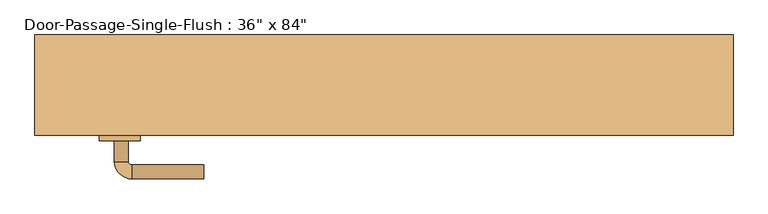
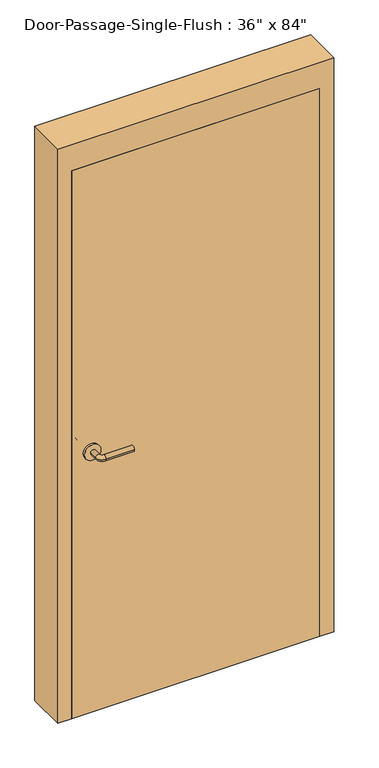
"""IFC4 building model written with IfcOpenShell, lengths in millimetres: door geometry."""

import ifcopenshell
import ifcopenshell.guid

model = None  # the IFC model being written
_history = None  # IfcOwnerHistory: only IFC2X3 demands one
_inside = {}  # id of a spatial element -> (the spatial element, [elements in it])
_under = {}  # id of a project, library or spatial element -> (it, [spatial elements below it])
_declared = {}  # id of a project -> (the project, [libraries it declares])
_typed = {}  # id of a type object -> (the type object, [elements of that type])
_made_of = {}  # id of a material, layer set ... -> (it, [elements and type objects made of it])


def new_model(schema):
    """Start an empty IFC model of exactly this schema.

    Asked for "IFC4X3", IfcOpenShell would pick the latest addendum, in which some entities
    have other attributes; the version numbers below select the first issue.
    IFC2X3 requires an IfcOwnerHistory on every rooted entity: one is made here for all.
    """
    global model, _history
    if schema == "IFC4X3":
        model = ifcopenshell.file(schema_version=(4, 3, 0, 0))
    else:
        model = ifcopenshell.file(schema=schema)
    _inside.clear()
    _under.clear()
    _declared.clear()
    _typed.clear()
    _made_of.clear()
    _history = None
    if model.schema == "IFC2X3":
        org = make("IfcOrganization", Name="unknown")
        user = make(
            "IfcPersonAndOrganization",
            ThePerson=make("IfcPerson", FamilyName="unknown"),
            TheOrganization=org,
        )
        app = make(
            "IfcApplication",
            ApplicationDeveloper=org,
            Version="unknown",
            ApplicationFullName="unknown",
            ApplicationIdentifier="unknown",
        )
        _history = make(
            "IfcOwnerHistory",
            OwningUser=user,
            OwningApplication=app,
            ChangeAction="ADDED",
            CreationDate=0,
        )
    return model


def make(cls, **values):
    """One entity of the class cls with the attributes given. An attribute that is None is left unset."""
    return model.create_entity(
        cls, **{name: value for name, value in values.items() if value is not None}
    )


def rooted(cls, **values):
    """An entity with a GlobalId (a new one), such as an element, a storey or a relation."""
    return make(cls, GlobalId=ifcopenshell.guid.new(), OwnerHistory=_history, **values)


def si_unit(unit_type, name, prefix=None):
    """IfcSIUnit, for example si_unit("LENGTHUNIT", "METRE", prefix="MILLI")."""
    return make("IfcSIUnit", UnitType=unit_type, Prefix=prefix, Name=name)


def assignment(units):
    """IfcUnitAssignment: the units of a project."""
    return None if units is None else make("IfcUnitAssignment", Units=units)


def point(xyz):
    """IfcCartesianPoint."""
    return None if xyz is None else make("IfcCartesianPoint", Coordinates=xyz)


def direction(xyz):
    """IfcDirection."""
    return None if xyz is None else make("IfcDirection", DirectionRatios=xyz)


def frame(location, z_axis=None, x_axis=None):
    """IfcAxis2Placement3D, a coordinate frame: its origin and axes. An axis left out is left unset."""
    return make(
        "IfcAxis2Placement3D",
        Location=point(location),
        Axis=direction(z_axis),
        RefDirection=direction(x_axis),
    )


def frame_2d(location, x_axis=None):
    """IfcAxis2Placement2D, a coordinate frame in the plane: its origin and x axis."""
    return make(
        "IfcAxis2Placement2D", Location=point(location), RefDirection=direction(x_axis)
    )


def origin():
    """The frame at (0, 0, 0) with its axes left unset."""
    return frame((0.0, 0.0, 0.0))


def origin_with_axes():
    """The frame at (0, 0, 0) with the z axis (0, 0, 1) and the x axis (1, 0, 0) written out."""
    return frame((0.0, 0.0, 0.0), z_axis=(0.0, 0.0, 1.0), x_axis=(1.0, 0.0, 0.0))


def place(relative_to, where):
    """IfcLocalPlacement: puts the frame where relative to a parent placement (None: the world)."""
    return make(
        "IfcLocalPlacement", PlacementRelTo=relative_to, RelativePlacement=where
    )


def context(
    kind, dimensions, precision=None, world=None, true_north=None, identifier=None
):
    """IfcGeometricRepresentationContext, for example the 3D "Model" context."""
    return make(
        "IfcGeometricRepresentationContext",
        ContextIdentifier=identifier,
        ContextType=kind,
        CoordinateSpaceDimension=dimensions,
        Precision=precision,
        WorldCoordinateSystem=world,
        TrueNorth=true_north,
    )


def project(units=None, contexts=None):
    """IfcProject with its units and contexts."""
    return rooted(
        "IfcProject",
        Name="project",
        RepresentationContexts=contexts,
        UnitsInContext=assignment(units),
    )


def spatial(cls, under=None, at=None, **own):
    """A site, building, storey or space (cls), placed at a placement, below another one or the project."""
    s = rooted(cls, ObjectPlacement=at, **own)
    if under is not None:
        _under.setdefault(under.id(), (under, []))[1].append(s)
    return s


def polyline(points):
    """IfcPolyline through the points."""
    return make("IfcPolyline", Points=[point(p) for p in points])


def circle_curve(where, radius):
    """IfcCircle in the frame where."""
    return make("IfcCircle", Position=where, Radius=radius)


def ellipse_curve(where, semi_axis1, semi_axis2):
    """IfcEllipse in the frame where."""
    return make(
        "IfcEllipse", Position=where, SemiAxis1=semi_axis1, SemiAxis2=semi_axis2
    )


def trimmed(basis, trim1, trim2, sense, master):
    """IfcTrimmedCurve: the piece of a basis curve between two trims."""
    return make(
        "IfcTrimmedCurve",
        BasisCurve=basis,
        Trim1=trim1,
        Trim2=trim2,
        SenseAgreement=sense,
        MasterRepresentation=master,
    )


def segment(curve, same_sense, transition):
    """IfcCompositeCurveSegment."""
    return make(
        "IfcCompositeCurveSegment",
        Transition=transition,
        SameSense=same_sense,
        ParentCurve=curve,
    )


def composite_curve(segments, self_intersect=None):
    """IfcCompositeCurve: segments joined end to end."""
    return make("IfcCompositeCurve", Segments=segments, SelfIntersect=self_intersect)


def outline(outer, holes=None, kind="AREA"):
    """IfcArbitraryClosedProfileDef: a profile drawn as a closed curve; with holes, ...WithVoids."""
    if holes is None:
        return make("IfcArbitraryClosedProfileDef", ProfileType=kind, OuterCurve=outer)
    return make(
        "IfcArbitraryProfileDefWithVoids",
        ProfileType=kind,
        OuterCurve=outer,
        InnerCurves=holes,
    )


def extrude(swept, where, along, depth):
    """IfcExtrudedAreaSolid: the profile swept, set in the frame where, extruded along a direction by depth."""
    return make(
        "IfcExtrudedAreaSolid",
        SweptArea=swept,
        Position=where,
        ExtrudedDirection=direction(along),
        Depth=depth,
    )


def faces_of(points, faces, orient=None, outer=None):
    """IfcFace entities. A face is a list of loops; a loop is a list of indices into points, from 0.

    orient and outer hold one flag for each loop. By default every Orientation is true, the
    first loop of a face is its IfcFaceOuterBound and the others are IfcFaceBound.
    """
    made = []
    for i, loops in enumerate(faces):
        bounds = []
        for j, loop in enumerate(loops):
            is_outer = j == 0 if outer is None else outer[i][j]
            bounds.append(
                make(
                    "IfcFaceOuterBound" if is_outer else "IfcFaceBound",
                    Bound=make("IfcPolyLoop", Polygon=[points[k] for k in loop]),
                    Orientation=True if orient is None else orient[i][j],
                )
            )
        made.append(make("IfcFace", Bounds=bounds))
    return made


def faceted_brep(points, faces, orient=None, outer=None, voids=None):
    """IfcFacetedBrep: a solid bounded by flat faces; with voids (closed shells), ...WithVoids."""
    shared = [point(p) for p in points]
    hull = make("IfcClosedShell", CfsFaces=faces_of(shared, faces, orient, outer))
    if voids is None:
        return make("IfcFacetedBrep", Outer=hull)
    return make(
        "IfcFacetedBrepWithVoids",
        Outer=hull,
        Voids=[
            make(cls, CfsFaces=faces_of(shared, fs, o, b)) for cls, fs, o, b in voids
        ],
    )


def shape(context_of_items, identifier, shape_type, items):
    """IfcShapeRepresentation: the items that make up one representation, for example the "Body"."""
    return make(
        "IfcShapeRepresentation",
        ContextOfItems=context_of_items,
        RepresentationIdentifier=identifier,
        RepresentationType=shape_type,
        Items=items,
    )


def source(mapping_origin, context_of_items, identifier, shape_type, items):
    """IfcRepresentationMap: a shape defined once, which mapped items show again and again."""
    return make(
        "IfcRepresentationMap",
        MappingOrigin=mapping_origin,
        MappedRepresentation=shape(context_of_items, identifier, shape_type, items),
    )


def transform(
    local_origin,
    x_axis=None,
    y_axis=None,
    z_axis=None,
    scale=None,
    scale2=None,
    scale3=None,
    uniform=True,
):
    """IfcCartesianTransformationOperator3D, or its non-uniform kind. x_axis, y_axis, z_axis: its Axis1, 2, 3."""
    if uniform:
        return make(
            "IfcCartesianTransformationOperator3D",
            Axis1=direction(x_axis),
            Axis2=direction(y_axis),
            LocalOrigin=point(local_origin),
            Scale=scale,
            Axis3=direction(z_axis),
        )
    return make(
        "IfcCartesianTransformationOperator3DnonUniform",
        Axis1=direction(x_axis),
        Axis2=direction(y_axis),
        LocalOrigin=point(local_origin),
        Scale=scale,
        Axis3=direction(z_axis),
        Scale2=scale2,
        Scale3=scale3,
    )


def mapped(mapping_source, mapping_target):
    """IfcMappedItem: shows the shape of a source again, moved by a transform."""
    return make(
        "IfcMappedItem", MappingSource=mapping_source, MappingTarget=mapping_target
    )


def made_of(thing, what):
    """Note that an element or type object is made of a material, layer set ...; save() writes the relation."""
    if what is not None:
        _made_of.setdefault(what.id(), (what, []))[1].append(thing)
    return thing


def element(
    cls,
    number,
    at=None,
    inside=None,
    cuts=None,
    type_object=None,
    material=None,
    context=None,
    identifier="Body",
    shape_type=None,
    held_by="IfcProductDefinitionShape",
    body=None,
    shapes=None,
    **own,
):
    """One element of the class cls, such as IfcWall. Its Tag is "e" and its number.

    at: its placement. inside: the storey or other place that contains it. cuts: it is an
    opening in that element (IfcRelVoidsElement). A single representation is given by context,
    identifier, shape_type and body (its items); several are given by shapes. held_by: the class
    of the entity that holds the representations. save() writes the other relations.
    """
    e = rooted(cls, Tag="e%d" % number, ObjectPlacement=at, **own)
    if body is not None:
        shapes = [shape(context, identifier, shape_type, body)]
    if shapes is not None:
        e.Representation = make(held_by, Representations=shapes)
    if inside is not None:
        _inside.setdefault(inside.id(), (inside, []))[1].append(e)
    if cuts is not None:
        rooted(
            "IfcRelVoidsElement", RelatingBuildingElement=cuts, RelatedOpeningElement=e
        )
    if type_object is not None:
        _typed.setdefault(type_object.id(), (type_object, []))[1].append(e)
    return made_of(e, material)


def aggregate(whole, parts):
    """IfcRelAggregates: a whole, such as a stair, and the parts it consists of."""
    return rooted("IfcRelAggregates", RelatingObject=whole, RelatedObjects=parts)


def save(model, path):
    """Write the relations noted so far, then the file.

    IfcRelAggregates (storeys below a building ...), IfcRelContainedInSpatialStructure (elements
    in a storey), IfcRelDefinesByType, IfcRelAssociatesMaterial and IfcRelDeclares: one each for
    every whole, place, type object, material and project.
    """
    for whole, parts in _under.values():
        aggregate(whole, parts)
    for where, things in _inside.values():
        rooted(
            "IfcRelContainedInSpatialStructure",
            RelatedElements=things,
            RelatingStructure=where,
        )
    for kind, things in _typed.values():
        rooted("IfcRelDefinesByType", RelatedObjects=things, RelatingType=kind)
    for what, things in _made_of.values():
        rooted("IfcRelAssociatesMaterial", RelatedObjects=things, RelatingMaterial=what)
    for by, libraries in _declared.values():
        rooted("IfcRelDeclares", RelatingContext=by, RelatedDefinitions=libraries)
    model.write(path)


def plane_surface(at):
    """IfcPlane: the flat surface through the origin of the frame at, square to its z axis."""
    return make("IfcPlane", Position=at)


def cylinder_surface(at, radius):
    """IfcCylindricalSurface: all points at the distance radius from the z axis of the frame at."""
    return make("IfcCylindricalSurface", Position=at, Radius=radius)


def revolved_surface(curve, axis_point, axis_direction):
    """IfcSurfaceOfRevolution: the curve turned about the line through axis_point along axis_direction."""
    return make(
        "IfcSurfaceOfRevolution",
        SweptCurve=make("IfcArbitraryOpenProfileDef", ProfileType="CURVE", Curve=curve),
        AxisPosition=make("IfcAxis1Placement", Location=point(axis_point), Axis=direction(axis_direction)),
    )


def advanced_brep(points, edges, surfaces, faces):
    """IfcAdvancedBrep: a solid bounded by faces that lie on surfaces and meet in shared edges.

    An edge is (start, end): straight between two places in points (the first is 0);
    or (start, end, curve); or (start, end, curve, False) where it runs against its curve.
    A face is (place in surfaces, loops), or (place, loops, False) where it looks against
    its surface's normal. A loop lists edges by number (the first is 1), with a minus sign
    where the edge is run from its end to its start. The first loop is the outer one.
    """
    corners = [point(p) for p in points]
    vertices = [make("IfcVertexPoint", VertexGeometry=c) for c in corners]
    made = []
    for start, end, *more in edges:
        made.append(
            make(
                "IfcEdgeCurve",
                EdgeStart=vertices[start],
                EdgeEnd=vertices[end],
                EdgeGeometry=more[0] if more else make("IfcPolyline", Points=[corners[start], corners[end]]),
                SameSense=more[1] if len(more) > 1 else True,
            )
        )
    hull = []
    for where, loops, *sense in faces:
        bounds = []
        for j, loop in enumerate(loops):
            ring = [make("IfcOrientedEdge", EdgeElement=made[abs(k) - 1], Orientation=k > 0) for k in loop]
            bounds.append(
                make(
                    "IfcFaceOuterBound" if j == 0 else "IfcFaceBound",
                    Bound=make("IfcEdgeLoop", EdgeList=ring),
                    Orientation=True,
                )
            )
        hull.append(make("IfcAdvancedFace", Bounds=bounds, FaceSurface=surfaces[where], SameSense=sense[0] if sense else True))
    return make("IfcAdvancedBrep", Outer=make("IfcClosedShell", CfsFaces=hull))


def door_01a91e93(model_context):
    return source(origin(), model_context, "Body", "SolidModel", [
        advanced_brep(
        [(-392.190625, -96.775, 1016.0), (-372.190625, -96.775, 1016.0), (-392.190625, -66.775, 1016.0), (-372.190625, -66.775, 1016.0), (-367.190625, -61.775, 1016.0), (-367.190625, -41.775, 1016.0), (-262.190625, -41.775, 1016.0), (-262.190625, -61.775, 1016.0)],
        [
            (0, 1, circle_curve(frame((-382.190625, -96.775, 1016.0), z_axis=(0.0, -1.0, 0.0), x_axis=(1.0, 0.0, 0.0)), 10.0)),
            (1, 0, circle_curve(frame((-382.190625, -96.775, 1016.0), z_axis=(0.0, -1.0, 0.0), x_axis=(1.0, 0.0, 0.0)), 10.0)),
            (0, 2),
            (2, 3, circle_curve(frame((-382.190625, -66.775, 1016.0), z_axis=(0.0, -1.0, 0.0), x_axis=(1.0, 0.0, 0.0)), 10.0)),
            (3, 1),
            (3, 2, circle_curve(frame((-382.190625, -66.775, 1016.0), z_axis=(0.0, -1.0, 0.0), x_axis=(1.0, 0.0, 0.0)), 10.0)),
            (4, 3, circle_curve(frame((-367.190625, -66.775, 1016.0), z_axis=(0.0, 0.0, 1.0), x_axis=(-1.0, 0.0, 0.0)), 5.0)),
            (2, 5, circle_curve(frame((-367.190625, -66.775, 1016.0), z_axis=(0.0, 0.0, -1.0), x_axis=(-1.0, 0.0, 0.0)), 25.0)),
            (5, 4, circle_curve(frame((-367.190625, -51.775, 1016.0), z_axis=(-1.0, 0.0, 0.0), x_axis=(0.0, -1.0, 0.0)), 10.0)),
            (4, 5, circle_curve(frame((-367.190625, -51.775, 1016.0), z_axis=(-1.0, 0.0, 0.0), x_axis=(0.0, -1.0, 0.0)), 10.0)),
            (6, 7, circle_curve(frame((-262.190625, -51.775, 1016.0), z_axis=(1.0, 0.0, 0.0), x_axis=(0.0, -1.0, 0.0)), 10.0)),
            (7, 6, circle_curve(frame((-262.190625, -51.775, 1016.0), z_axis=(1.0, 0.0, 0.0), x_axis=(0.0, -1.0, 0.0)), 10.0)),
            (5, 6),
            (7, 4),
        ],
        [
            plane_surface(frame((-382.190625, -96.775, 1016.0), z_axis=(0.0, -1.0, 0.0), x_axis=(0.0, 0.0, 1.0))),
            cylinder_surface(frame((-382.190625, -96.775, 1016.0), z_axis=(0.0, -1.0, 0.0), x_axis=(1.0, 0.0, 0.0)), 10.0),
            revolved_surface(trimmed(ellipse_curve(frame((-382.190625, -66.775, 1016.0), z_axis=(0.0, -1.0, 0.0), x_axis=(1.0, 0.0, 0.0)), 10.0, 10.0), [point((-392.190625, -66.775, 1016.0))], [point((-372.190625, -66.775, 1016.0))], True, "CARTESIAN"), (-367.190625, -66.775, 1016.0), (0.0, 0.0, -1.0)),
            revolved_surface(trimmed(ellipse_curve(frame((-382.190625, -66.775, 1016.0), z_axis=(0.0, -1.0, 0.0), x_axis=(1.0, 0.0, 0.0)), 10.0, 10.0), [point((-372.190625, -66.775, 1016.0))], [point((-392.190625, -66.775, 1016.0))], True, "CARTESIAN"), (-367.190625, -66.775, 1016.0), (0.0, 0.0, -1.0)),
            plane_surface(frame((-262.190625, -51.775, 1016.0), z_axis=(1.0, 0.0, 0.0), x_axis=(0.0, 0.0, 1.0))),
            cylinder_surface(frame((-367.190625, -51.775, 1016.0), z_axis=(-1.0, 0.0, 0.0), x_axis=(0.0, -1.0, 0.0)), 10.0),
        ],
        [
            (0, [[1, 2]]),
            (1, [[-1, 3, 4, 5]]),
            (1, [[-2, -5, 6, -3]]),
            (2, [[7, -4, 8, 9]]),
            (3, [[-8, -6, -7, 10]]),
            (4, [[11, 12]]),
            (5, [[-9, 13, -12, 14]]),
            (5, [[-10, -14, -11, -13]]),
        ],
    ),
        extrude(outline(composite_curve([segment(trimmed(circle_curve(frame_2d((1016.0, -384.690625)), 30.0), [point((1016.0, -414.690625))], [point((1016.0, -354.690625))], False, "CARTESIAN"), True, "CONTINUOUS"), segment(trimmed(circle_curve(frame_2d((1016.0, -384.690625)), 30.0), [point((1016.0, -354.690625))], [point((1016.0, -414.690625))], False, "CARTESIAN"), True, "CONTINUOUS")], self_intersect=False)), frame((0.0, -104.775, 0.0), z_axis=(0.0, 1.0, 0.0), x_axis=(0.0, 0.0, 1.0)), (0.0, 0.0, 1.0), 8.0),
        advanced_brep(
        [(-392.190625, -157.225, 1016.0), (-372.190625, -157.225, 1016.0), (-372.190625, -187.225, 1016.0), (-392.190625, -187.225, 1016.0), (-367.190625, -192.225, 1016.0), (-367.190625, -212.225, 1016.0), (-262.190625, -212.225, 1016.0), (-262.190625, -192.225, 1016.0)],
        [
            (0, 1, circle_curve(frame((-382.190625, -157.225, 1016.0), z_axis=(0.0, 1.0, 0.0), x_axis=(1.0, 0.0, 0.0)), 10.0)),
            (1, 0, circle_curve(frame((-382.190625, -157.225, 1016.0), z_axis=(0.0, 1.0, 0.0), x_axis=(1.0, 0.0, 0.0)), 10.0)),
            (1, 2),
            (2, 3, circle_curve(frame((-382.190625, -187.225, 1016.0), z_axis=(0.0, 1.0, 0.0), x_axis=(1.0, 0.0, 0.0)), 10.0)),
            (3, 0),
            (3, 2, circle_curve(frame((-382.190625, -187.225, 1016.0), z_axis=(0.0, 1.0, 0.0), x_axis=(1.0, 0.0, 0.0)), 10.0)),
            (4, 5, circle_curve(frame((-367.190625, -202.225, 1016.0), z_axis=(-1.0, 0.0, 0.0), x_axis=(0.0, 1.0, 0.0)), 10.0)),
            (5, 3, circle_curve(frame((-367.190625, -187.225, 1016.0), z_axis=(0.0, 0.0, -1.0), x_axis=(-1.0, 0.0, 0.0)), 25.0)),
            (2, 4, circle_curve(frame((-367.190625, -187.225, 1016.0), z_axis=(0.0, 0.0, 1.0), x_axis=(-1.0, 0.0, 0.0)), 5.0)),
            (5, 4, circle_curve(frame((-367.190625, -202.225, 1016.0), z_axis=(-1.0, 0.0, 0.0), x_axis=(0.0, 1.0, 0.0)), 10.0)),
            (6, 7, circle_curve(frame((-262.190625, -202.225, 1016.0), z_axis=(1.0, 0.0, 0.0), x_axis=(0.0, 1.0, 0.0)), 10.0)),
            (7, 6, circle_curve(frame((-262.190625, -202.225, 1016.0), z_axis=(1.0, 0.0, 0.0), x_axis=(0.0, 1.0, 0.0)), 10.0)),
            (4, 7),
            (6, 5),
        ],
        [
            plane_surface(frame((-382.190625, -157.225, 1016.0), z_axis=(0.0, 1.0, 0.0), x_axis=(0.0, 0.0, 1.0))),
            cylinder_surface(frame((-382.190625, -157.225, 1016.0), z_axis=(0.0, 1.0, 0.0), x_axis=(1.0, 0.0, 0.0)), 10.0),
            revolved_surface(trimmed(ellipse_curve(frame((-382.190625, -187.225, 1016.0), z_axis=(0.0, -1.0, 0.0), x_axis=(1.0, 0.0, 0.0)), 10.0, 10.0), [point((-392.190625, -187.225, 1016.0))], [point((-372.190625, -187.225, 1016.0))], True, "CARTESIAN"), (-367.190625, -187.225, 1016.0), (0.0, 0.0, -1.0)),
            revolved_surface(trimmed(ellipse_curve(frame((-382.190625, -187.225, 1016.0), z_axis=(0.0, -1.0, 0.0), x_axis=(1.0, 0.0, 0.0)), 10.0, 10.0), [point((-372.190625, -187.225, 1016.0))], [point((-392.190625, -187.225, 1016.0))], True, "CARTESIAN"), (-367.190625, -187.225, 1016.0), (0.0, 0.0, -1.0)),
            plane_surface(frame((-262.190625, -202.225, 1016.0), z_axis=(1.0, 0.0, 0.0), x_axis=(0.0, 0.0, 1.0))),
            cylinder_surface(frame((-367.190625, -202.225, 1016.0), z_axis=(-1.0, 0.0, 0.0), x_axis=(0.0, 1.0, 0.0)), 10.0),
        ],
        [
            (0, [[1, 2]]),
            (1, [[3, 4, 5, -2]]),
            (1, [[-5, 6, -3, -1]]),
            (2, [[7, 8, -4, 9]]),
            (3, [[10, -9, -6, -8]]),
            (4, [[11, 12]]),
            (5, [[13, -11, 14, -7]]),
            (5, [[-14, -12, -13, -10]]),
        ],
    ),
        extrude(outline(composite_curve([segment(trimmed(circle_curve(frame_2d((1016.0, -384.690625)), 30.0), [point((1016.0, -414.690625))], [point((1016.0, -354.690625))], False, "CARTESIAN"), True, "CONTINUOUS"), segment(trimmed(circle_curve(frame_2d((1016.0, -384.690625)), 30.0), [point((1016.0, -354.690625))], [point((1016.0, -414.690625))], False, "CARTESIAN"), True, "CONTINUOUS")], self_intersect=False)), frame((0.0, -157.225, 0.0), z_axis=(0.0, 1.0, 0.0), x_axis=(0.0, 0.0, 1.0)), (0.0, 0.0, 1.0), 8.0),
        faceted_brep([(457.2, -100.0125, 0.0), (441.325, -100.0125, 0.0), (441.325, -52.3875, 0.0), (457.2, -52.3875, 0.0), (457.2, -3.175, 0.0), (508.0, -3.175, 0.0), (508.0, -149.225, 0.0), (457.2, -149.225, 0.0), (457.2, -149.225, 2133.6), (457.2, -100.0125, 2133.6), (508.0, -149.225, 2235.2), (-508.0, -149.225, 2235.2), (-508.0, -149.225, 0.0), (-457.2, -149.225, 0.0), (-457.2, -149.225, 2133.6), (508.0, -3.175, 2235.2), (457.2, -3.175, 2133.6), (-457.2, -3.175, 2133.6), (-457.2, -3.175, 0.0), (-508.0, -3.175, 0.0), (-508.0, -3.175, 2235.2), (457.2, -52.3875, 2133.6), (441.325, -52.3875, 2117.725), (-441.325, -52.3875, 2117.725), (-441.325, -52.3875, 0.0), (-457.2, -52.3875, 0.0), (-457.2, -52.3875, 2133.6), (441.325, -100.0125, 2117.725), (-457.2, -100.0125, 2133.6), (-457.2, -100.0125, 0.0), (-441.325, -100.0125, 0.0), (-441.325, -100.0125, 2117.725)], [[[0, 1, 2, 3, 4, 5, 6, 7]], [[7, 8, 9, 0]], [[6, 10, 11, 12, 13, 14, 8, 7]], [[5, 15, 10, 6]], [[4, 16, 17, 18, 19, 20, 15, 5]], [[3, 21, 16, 4]], [[2, 22, 23, 24, 25, 26, 21, 3]], [[1, 27, 22, 2]], [[0, 9, 28, 29, 30, 31, 27, 1]], [[8, 14, 28, 9]], [[16, 21, 26, 17]], [[22, 27, 31, 23]], [[12, 19, 18, 25, 24, 30, 29, 13]], [[13, 29, 28, 14]], [[11, 20, 19, 12]], [[17, 26, 25, 18]], [[23, 31, 30, 24]], [[15, 20, 11, 10]]]),
        extrude(outline(polyline([(457.2, -104.775), (457.2, -149.225), (-457.2, -149.225), (-457.2, -104.775), (457.2, -104.775)])), origin_with_axes(), (0.0, 0.0, 1.0), 2133.6),
    ])


if __name__ == "__main__":
    model = new_model("IFC4")
    model_context = context("Model", 3, world=origin())
    ifc_project = project(units=[si_unit("LENGTHUNIT", "METRE", prefix="MILLI")], contexts=[model_context])
    site = spatial("IfcSite", under=ifc_project)
    building = spatial("IfcBuilding", under=site)
    placement = place(None, origin())
    door_shape = door_01a91e93(model_context)
    element("IfcDoor", 1, ObjectType="Door-Passage-Single-Flush : 36\" x 84\"", at=placement, inside=building, context=model_context, shape_type="MappedRepresentation", body=[
        mapped(door_shape, transform((0.0, 0.0, 0.0), x_axis=(1.0, 0.0, 0.0), y_axis=(0.0, 1.0, 0.0), z_axis=(0.0, 0.0, 1.0))),
    ])
    save(model, "model.ifc")

# Revit data of these elements
# Type "Door-Passage-Single-Flush : 36\" x 84\""
#   Type Mark = "1"
#   Assembly Code = "B2030200"
#   Analytic Construction = "Wooden"
#   Thickness = 0' - 1 3/4"
#   Thermal Resistance (R) = 2.5876 (h·ft²·°F)/BTU
#   Swing Angle [instance default] = 90.00°
#   Strike Height = 3' - 4"
#   Rough Width [instance default] = 3' - 4"
#   Rough Height [instance default] = 7' - 4"
#   MF Opening Height [instance default] = 0' - 4"
#   MF Opening Width [instance default] = 0' - 4"
#   Inset Calculate [instance default] = 0' - 4"
#   Masonry Inset [instance default] = 0' - 1"
#   Height = 7' - 0"
#   Width = 3' - 0"
#   Heat Transfer Coefficient (U) = 0.3865 BTU/(h·ft²·°F)
#   Masonry Frame Depth = 0' - 5 3/4"
#   Define Thermal Properties by = 1
#   Masonry Frame [instance default] = yes
#   Function = 1
#   Dry Wall Frame [instance default] = no
#   Panel Material = Wood - Birch
#   Frame Material = Metal - Paint Finish - Grey
#   Door Handle Material = Aluminum
#   Visual Light Transmittance = 0
#   Solar Heat Gain Coefficient = 0
#   Wall Closure = (empty or 0)
# Element 1 (IfcDoor, "Door-Passage-Single-Flush : 36\" x 84\"")
#   Materials on its faces: "Aluminum", "Metal - Paint Finish - Grey", "Wood - Birch"
# Materials
#   "Wood - Birch": class "Wood", colour RGB 166 116 52, transparency 0, Cost = 0
#   "Metal - Paint Finish - Grey": class "Paint", colour RGB 104 104 104, transparency 0, Cost = 0
#   "Aluminum": class "Metal", colour RGB 247 247 247, transparency 0, Description = "Aluminum 6061", Cost = 0
